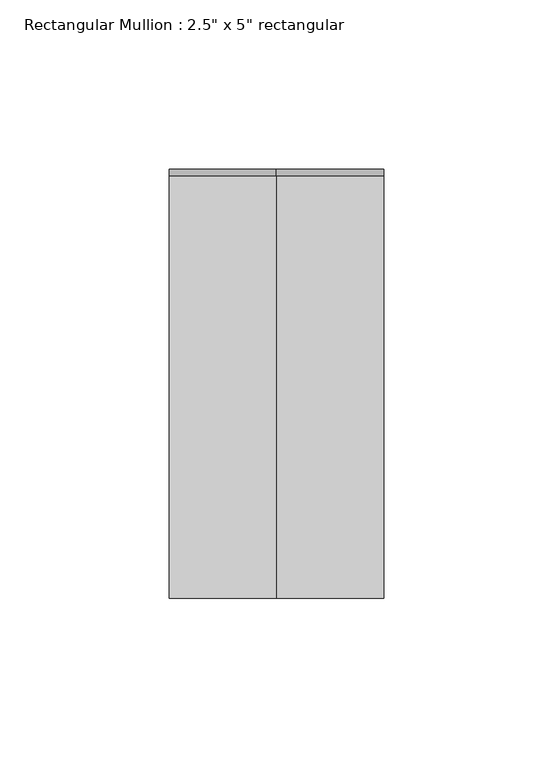
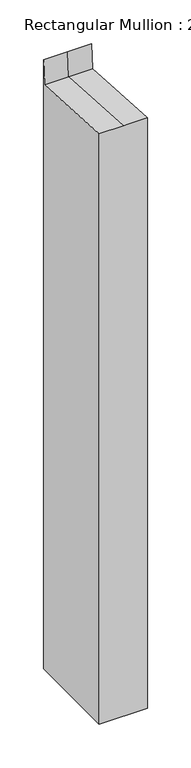
"""IFC4 building model written with IfcOpenShell, lengths in millimetres: member geometry."""

from ifc_helpers import new_model, si_unit, origin, place, context, project, spatial, faceted_brep, source, transform, mapped, element, save


def member_1fc1b455(model_context):
    return source(origin(), model_context, "Body", "Brep", [
        faceted_brep([(31.75, 63.5, -819.15), (31.75, -63.5, -819.15), (-31.75, -63.5, -819.15), (-31.75, 63.5, -819.15), (-31.75, 63.5, 29.7846233), (0.0, 63.5, 29.7846233), (31.75, 63.5, 29.7846233), (-31.75, -63.5, 3.8736342), (-31.75, 61.4149606, -3.8662198), (31.75, -63.5, 3.8736342), (0.0, -63.5, 3.8736342), (31.75, 61.4149606, -3.8662198), (0.0, 61.4149606, -3.8662198)], [[[0, 1, 2, 3]], [[4, 5, 6, 0, 3]], [[7, 8, 4, 3, 2]], [[9, 10, 7, 2, 1]], [[6, 11, 9, 1, 0]], [[6, 5, 12, 11]], [[5, 4, 8, 12]], [[8, 7, 10, 12]], [[10, 9, 11, 12]]]),
    ])


if __name__ == "__main__":
    model = new_model("IFC4")
    model_context = context("Model", 3, world=origin())
    ifc_project = project(units=[si_unit("LENGTHUNIT", "METRE", prefix="MILLI")], contexts=[model_context])
    site = spatial("IfcSite", under=ifc_project)
    building = spatial("IfcBuilding", under=site)
    placement = place(None, origin())
    member_shape = member_1fc1b455(model_context)
    element("IfcMember", 1, ObjectType="Rectangular Mullion : 2.5\" x 5\" rectangular", at=placement, inside=building, context=model_context, shape_type="MappedRepresentation", body=[
        mapped(member_shape, transform((0.0, 0.0, 0.0), x_axis=(1.0, 0.0, 0.0), y_axis=(0.0, 1.0, 0.0), z_axis=(0.0, 0.0, 1.0))),
    ])
    save(model, "model.ifc")

# Revit data of these elements
# Type "Rectangular Mullion : 2.5\" x 5\" rectangular"
#   built-in parameter 1007304 = 0.416667 (stored number, unit not read)
#   built-in parameter 1007301 = 0.104167 (stored number, unit not read)
#   built-in parameter 1007300 = 0.104167 (stored number, unit not read)
# Element 1 (IfcMember, "Rectangular Mullion : 2.5\" x 5\" rectangular")
#   Materials on its faces: "Metal - Aluminum"
# Materials
#   "Metal - Aluminum": class "Metal", colour RGB 247 247 247, transparency 0, Cost = 0
